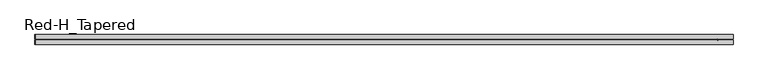
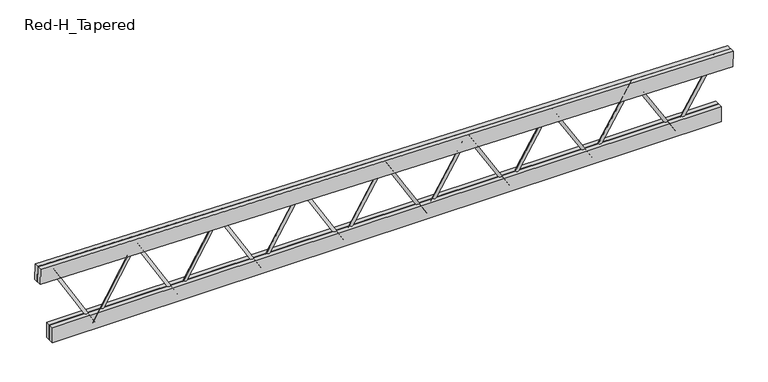
"""IFC4 building model written with IfcOpenShell, lengths in millimetres: beam geometry, Construction_Frames_RedBuilt_Openweb_Red-H_Tapered : Red-H_Tapered."""

from ifc_helpers import new_model, si_unit, point, frame, origin, origin_2d, place, context, project, spatial, polyline, circle_curve, trimmed, segment, composite_curve, outline, extrude, source, transform, mapped, element, save


def red_h_tapered_fac266aa(model_context):
    return source(origin(), model_context, "Body", "SweptSolid", [
        extrude(outline(composite_curve([segment(trimmed(circle_curve(origin_2d(), 12.7), [point((0.0, 12.7))], [point((0.0, -12.7))], False, "CARTESIAN"), True, "CONTINUOUS"), segment(trimmed(circle_curve(origin_2d(), 12.7), [point((0.0, -12.7))], [point((0.0, 12.7))], False, "CARTESIAN"), True, "CONTINUOUS")], self_intersect=False)), frame((2515.0014939, 0.0, -367.0101562), z_axis=(0.5238628746877177, 0.0, 0.8518026112450705), x_axis=(0.0, -1.0, 0.0)), (0.0, 0.0, 1.0), 685.8396444),
        extrude(outline(composite_curve([segment(trimmed(circle_curve(origin_2d(), 12.7), [point((0.0, -12.7000001))], [point((0.0, 12.7))], False, "CARTESIAN"), True, "CONTINUOUS"), segment(trimmed(circle_curve(origin_2d(), 12.7), [point((0.0, 12.7))], [point((0.0, -12.7000001))], False, "CARTESIAN"), True, "CONTINUOUS")], self_intersect=False)), frame((2515.0014939, 0.0, -367.0101562), z_axis=(-0.521291788288458, 0.0, 0.8533785042189788), x_axis=(0.0, -1.0, 0.0)), (0.0, 0.0, 1.0), 689.2223046),
        extrude(outline(composite_curve([segment(trimmed(circle_curve(origin_2d(), 12.7), [point((0.0, 12.7))], [point((0.0, -12.7))], False, "CARTESIAN"), True, "CONTINUOUS"), segment(trimmed(circle_curve(origin_2d(), 12.7), [point((0.0, -12.7))], [point((0.0, 12.7))], False, "CARTESIAN"), True, "CONTINUOUS")], self_intersect=False)), frame((1796.4296385, 0.0, -367.0101562), z_axis=(0.5212917882884571, 0.0, 0.8533785042189793), x_axis=(0.0, -1.0, 0.0)), (0.0, 0.0, 1.0), 689.2223046),
        extrude(outline(composite_curve([segment(trimmed(circle_curve(origin_2d(), 12.7), [point((0.0, -12.7000001))], [point((0.0, 12.6999999))], False, "CARTESIAN"), True, "CONTINUOUS"), segment(trimmed(circle_curve(origin_2d(), 12.7), [point((0.0, 12.6999999))], [point((0.0, -12.7000001))], False, "CARTESIAN"), True, "CONTINUOUS")], self_intersect=False)), frame((1796.4296385, 0.0, -367.0101562), z_axis=(-0.5187411676162772, 0.0, 0.8549313428691812), x_axis=(0.0, -1.0, 0.0)), (0.0, 0.0, 1.0), 692.6111713),
        extrude(outline(composite_curve([segment(trimmed(circle_curve(origin_2d(), 12.7), [point((0.0, 12.7))], [point((0.0, -12.7))], False, "CARTESIAN"), True, "CONTINUOUS"), segment(trimmed(circle_curve(origin_2d(), 12.7), [point((0.0, -12.7))], [point((0.0, 12.7))], False, "CARTESIAN"), True, "CONTINUOUS")], self_intersect=False)), frame((1077.8577831, 0.0, -367.0101562), z_axis=(0.5187411676162762, 0.0, 0.8549313428691818), x_axis=(0.0, -1.0, 0.0)), (0.0, 0.0, 1.0), 692.6111713),
        extrude(outline(composite_curve([segment(trimmed(circle_curve(origin_2d(), 12.7), [point((0.0, -12.7))], [point((0.0, 12.7))], False, "CARTESIAN"), True, "CONTINUOUS"), segment(trimmed(circle_curve(origin_2d(), 12.7), [point((0.0, 12.7))], [point((0.0, -12.7))], False, "CARTESIAN"), True, "CONTINUOUS")], self_intersect=False)), frame((1077.8577831, 0.0, -367.0101562), z_axis=(-0.516210849200197, 0.0, 0.8564615339686958), x_axis=(0.0, -1.0, 0.0)), (0.0, 0.0, 1.0), 696.0061538),
        extrude(outline(composite_curve([segment(trimmed(circle_curve(origin_2d(), 12.7), [point((0.0, 12.7))], [point((0.0, -12.7))], False, "CARTESIAN"), True, "CONTINUOUS"), segment(trimmed(circle_curve(origin_2d(), 12.7), [point((0.0, -12.7))], [point((0.0, 12.7))], False, "CARTESIAN"), True, "CONTINUOUS")], self_intersect=False)), frame((359.2859277, 0.0, -367.0101562), z_axis=(0.5162108492001977, 0.0, 0.8564615339686954), x_axis=(0.0, -1.0, 0.0)), (0.0, 0.0, 1.0), 696.0061538),
        extrude(outline(composite_curve([segment(trimmed(circle_curve(origin_2d(), 12.7), [point((0.0, -12.7))], [point((0.0, 12.6999999))], False, "CARTESIAN"), True, "CONTINUOUS"), segment(trimmed(circle_curve(origin_2d(), 12.7), [point((0.0, 12.6999999))], [point((0.0, -12.7))], False, "CARTESIAN"), True, "CONTINUOUS")], self_intersect=False)), frame((359.2859277, 0.0, -367.0101562), z_axis=(-0.5137006691841284, 0.0, 0.857969476426626), x_axis=(0.0, -1.0, 0.0)), (0.0, 0.0, 1.0), 699.4071631),
        extrude(outline(composite_curve([segment(trimmed(circle_curve(origin_2d(), 12.7), [point((0.0, -12.6999999))], [point((0.0, 12.7))], False, "CARTESIAN"), True, "CONTINUOUS"), segment(trimmed(circle_curve(origin_2d(), 12.7), [point((0.0, 12.7))], [point((0.0, -12.6999999))], False, "CARTESIAN"), True, "CONTINUOUS")], self_intersect=False)), frame((-359.2859277, 0.0, -367.0101562), z_axis=(0.5137006691840971, 0.0, 0.8579694764266448), x_axis=(0.0, -1.0, 0.0)), (0.0, 0.0, 1.0), 699.4071631),
        extrude(outline(composite_curve([segment(trimmed(circle_curve(origin_2d(), 12.7), [point((0.0, 12.6999999))], [point((0.0, -12.7))], False, "CARTESIAN"), True, "CONTINUOUS"), segment(trimmed(circle_curve(origin_2d(), 12.7), [point((0.0, -12.7))], [point((0.0, 12.6999999))], False, "CARTESIAN"), True, "CONTINUOUS")], self_intersect=False)), frame((-359.2859277, 0.0, -367.0101562), z_axis=(-0.5112104634271143, 0.0, 0.8594555614356307), x_axis=(0.0, -1.0, 0.0)), (0.0, 0.0, 1.0), 702.8141116),
        extrude(outline(composite_curve([segment(trimmed(circle_curve(origin_2d(), 12.7), [point((0.0, -12.6999999))], [point((0.0, 12.7000001))], False, "CARTESIAN"), True, "CONTINUOUS"), segment(trimmed(circle_curve(origin_2d(), 12.7), [point((0.0, 12.7000001))], [point((0.0, -12.6999999))], False, "CARTESIAN"), True, "CONTINUOUS")], self_intersect=False)), frame((-1077.8577831, 0.0, -367.0101562), z_axis=(0.5112104634271127, 0.0, 0.8594555614356316), x_axis=(0.0, -1.0, 0.0)), (0.0, 0.0, 1.0), 702.8141116),
        extrude(outline(composite_curve([segment(trimmed(circle_curve(origin_2d(), 12.7), [point((0.0, 12.7))], [point((0.0, -12.7))], False, "CARTESIAN"), True, "CONTINUOUS"), segment(trimmed(circle_curve(origin_2d(), 12.7), [point((0.0, -12.7))], [point((0.0, 12.7))], False, "CARTESIAN"), True, "CONTINUOUS")], self_intersect=False)), frame((-1077.8577831, 0.0, -367.0101562), z_axis=(-0.5087400675988082, 0.0, 0.8609201726173921), x_axis=(0.0, -1.0, 0.0)), (0.0, 0.0, 1.0), 706.2269135),
        extrude(outline(composite_curve([segment(trimmed(circle_curve(origin_2d(), 12.7), [point((0.0, -12.7))], [point((0.0, 12.7))], False, "CARTESIAN"), True, "CONTINUOUS"), segment(trimmed(circle_curve(origin_2d(), 12.7), [point((0.0, 12.7))], [point((0.0, -12.7))], False, "CARTESIAN"), True, "CONTINUOUS")], self_intersect=False)), frame((-1796.4296385, 0.0, -367.0101562), z_axis=(0.5087400675988213, 0.0, 0.8609201726173843), x_axis=(0.0, -1.0, 0.0)), (0.0, 0.0, 1.0), 706.2269135),
        extrude(outline(composite_curve([segment(trimmed(circle_curve(origin_2d(), 12.7), [point((0.0, 12.7))], [point((0.0, -12.7))], False, "CARTESIAN"), True, "CONTINUOUS"), segment(trimmed(circle_curve(origin_2d(), 12.7), [point((0.0, -12.7))], [point((0.0, 12.7))], False, "CARTESIAN"), True, "CONTINUOUS")], self_intersect=False)), frame((-1796.4296385, 0.0, -367.0101562), z_axis=(-0.5062893172698196, 0.0, 0.8623636861663762), x_axis=(0.0, -1.0, 0.0)), (0.0, 0.0, 1.0), 709.6454842),
        extrude(outline(composite_curve([segment(trimmed(circle_curve(origin_2d(), 12.7), [point((0.0, -12.7))], [point((0.0, 12.7000001))], False, "CARTESIAN"), True, "CONTINUOUS"), segment(trimmed(circle_curve(origin_2d(), 12.7), [point((0.0, 12.7000001))], [point((0.0, -12.7))], False, "CARTESIAN"), True, "CONTINUOUS")], self_intersect=False)), frame((-2515.0014939, 0.0, -367.0101562), z_axis=(0.506289317269808, 0.0, 0.862363686166383), x_axis=(0.0, -1.0, 0.0)), (0.0, 0.0, 1.0), 709.6454842),
        extrude(outline(composite_curve([segment(trimmed(circle_curve(origin_2d(), 12.7), [point((0.0, 12.7))], [point((0.0, -12.7))], False, "CARTESIAN"), True, "CONTINUOUS"), segment(trimmed(circle_curve(origin_2d(), 12.7), [point((0.0, -12.7))], [point((0.0, 12.7))], False, "CARTESIAN"), True, "CONTINUOUS")], self_intersect=False)), frame((-2515.0014939, 0.0, -367.0101562), z_axis=(-0.5038580479976326, 0.0, 0.8637864709915382), x_axis=(0.0, -1.0, 0.0)), (0.0, 0.0, 1.0), 713.0697408),
        extrude(outline(polyline([(-2899.6874215, -41.275), (-2899.6874215, -3.175), (2899.6874215, -3.175), (2899.6874215, -41.275), (-2899.6874215, -41.275)])), frame((0.0, 0.0, -386.0601562), z_axis=(0.0, 0.0, 1.0), x_axis=(1.0, 0.0, 0.0)), (0.0, 0.0, 1.0), 139.7),
        extrude(outline(polyline([(-2899.6874215, 3.175), (-2899.6874215, 41.275), (2899.6874215, 41.275), (2899.6874215, 3.175), (-2899.6874215, 3.175)])), frame((0.0, 0.0, -386.0601562), z_axis=(0.0, 0.0, 1.0), x_axis=(1.0, 0.0, 0.0)), (0.0, 0.0, 1.0), 139.7),
        extrude(outline(polyline([(0.0, -38.1), (0.0, 0.0), (6003.4346259, 0.0), (6003.4346259, -38.1), (0.0, -38.1)])), frame((-3003.6516548, -3.175, 185.4598509), z_axis=(0.01692364560154581, 0.0, 0.9998567848544877), x_axis=(0.9998567848544877, 0.0, -0.01692364560154581)), (0.0, 0.0, 1.0), 139.7),
        extrude(outline(polyline([(0.0, -38.1), (0.0, 0.0), (6003.4346259, 0.0), (6003.4346259, -38.1), (0.0, -38.1)])), frame((-3003.6516548, 41.275, 185.4598509), z_axis=(0.01692364560154581, 0.0, 0.9998567848544877), x_axis=(0.9998567848544877, 0.0, -0.01692364560154581)), (0.0, 0.0, 1.0), 139.7),
    ])


if __name__ == "__main__":
    model = new_model("IFC4")
    model_context = context("Model", 3, world=origin())
    ifc_project = project(units=[si_unit("LENGTHUNIT", "METRE", prefix="MILLI")], contexts=[model_context])
    site = spatial("IfcSite", under=ifc_project)
    building = spatial("IfcBuilding", under=site)
    placement = place(None, origin())
    red_h_tapered_shape = red_h_tapered_fac266aa(model_context)
    element("IfcBeam", 1, ObjectType="Construction_Frames_RedBuilt_Openweb_Red-H_Tapered : Red-H_Tapered", at=placement, inside=building, context=model_context, shape_type="MappedRepresentation", body=[
        mapped(red_h_tapered_shape, transform((0.0, 0.0, 0.0), x_axis=(1.0, 0.0, 0.0), y_axis=(0.0, 1.0, 0.0), z_axis=(0.0, 0.0, 1.0))),
    ])
    save(model, "model.ifc")

# Revit data of these elements
# Type "Construction_Frames_RedBuilt_Openweb_Red-H_Tapered : Red-H_Tapered"
#   Youtube clip = ""
#   Weight Net (Kg) = "0"
#   Webs = "Up to 2\" diameter tubular steel"
#   Uniformat II Description = ""
#   Uniformat II Code = ""
#   Uniclass 2015 Name = "Softwood trusses"
#   Uniclass 2015 Code = "Pr_20_85_90_81"
#   Uniclass 2.0 Description = "Structural Framing Systems"
#   Uniclass 2.0 Code = "SS-15-10-75"
#   Uniclass 1.4 Description = "Trusses"
#   Uniclass 1.4 Code = "L3523"
#   UNSPSC Code = "30103606"
#   Technical description = "http://www.redbuilt.com/reference/literature-and-other-resources"
#   Region South America = "None"
#   Region Oceania = "None"
#   Region North America = "US"
#   Region Middle East = "None"
#   Region Europe = "None"
#   Region Asia = "None"
#   Region Antarctica = "None"
#   Region Africa = "None"
#   QR code = "http://bimobject.com/redbuilt/product/redbuilt-0003"
#   Product url = "http://www.redbuilt.com/products/default.aspx?id=2"
#   Product group = "Wood Trusses"
#   Product family = "Construction"
#   Product data url = "https://bimobject.com/redbuilt/product/redbuilt-0003"
#   Product certification = ""
#   Product SKU = "redbuilt-0003"
#   Product Page URL = "http://www.redbuilt.com/commercial-systems/red-m-red-h-open-web-trusses"
#   Product Guid = "2c5793f2-6ffb-4665-b825-cf90c048e711"
#   Product Documentation Link = "http://www.redbuilt.com/documents/OW_Guide_2017_07_LowRes_wLinks.pdf"
#   OmniClass Description = "Wood Trusses"
#   OmniClass Code = "23-13 35 19 13 17"
#   NBS Reference Description = ""
#   NBS Reference Code = ""
#   Material secondary = "Steel"
#   Material main = "CHARRED WOOD"
#   Masterformat 2014 Description = "Metal-Web Wood Joists"
#   Masterformat 2014 Code = "06 17 36"
#   Manufacturer name = "RedBuilt"
#   Manufacturer country = "United States"
#   Installation instructions = "http://www.redbuilt.com/documents/Installation_Sheets_Open-Web.pdf"
#   IFC Classification = ""
#   EAN code = ""
#   Design country = "United States"
#   Product Information = "http://redbuilt.com/products/default.aspx?id=2"
#   Model = "Red-H-Tapered"
#   Manufacturer URL = "http://redbuilt.com/"
#   Manufacturer = "RedBuilt™"
#   Description = "Open Web Truss"
#   Date of publishing = "8/17/2010"
#   Contact us = "http://redbuilt.com/contact/"
#   Chords = "Double 1½\" x 5½\" MSR lumber"
#   COBIe Type Category = ""
#   Brand url = "http://www.redbuilt.com"
#   BIMobject main category code = "construction"
#   BIMobject main category = "Construction"
#   BIMobject category code = "construction-frames-trusses"
#   BIMobject category = "Frames & Trusses"
#   Web Radius = 0' - 0 1/2"
#   Web Layout Offset Start [instance default] = 0' - 5"
#   Web Layout Offset End [instance default] = 0' - 5"
#   Web Diameter = 0' - 1"
#   TotalLength [instance default] = 20' - 0"
#   Span Minimum = 4' - 0"
#   Span Maximum = 70' - 0"
#   Span Limit [instance default] = 20' - 0"
#   Nominal width = 0' - 0"
#   Nominal height = 0' - 0"
#   Inner Depth Top [instance default] = 0' - 2.76372"
#   Depth Start [instance default] = 6' - 0"
#   Top Chord Length [instance default] = 20' - 1.19701"
#   TC Extension Start Aux [instance default] = 0' - 0"
#   TC Extension End Aux [instance default] = 0' - 0"
#   T-B Chord Length Difference L [instance default] = 0' - 4"
#   T-B Chord Length Difference [instance default] = 0' - 4"
#   Height 2 [instance default] = 6' - 0"
#   Depth Minimum at Wall = 2' - 0"
#   Depth Maximum at Wall = 6' - 0"
#   Depth Lower End [instance default] = 2' - 0"
#   Depth Higher End [instance default] = 6' - 0"
#   Depth End [instance default] = 2' - 0"
#   Depth 2 [instance default] = 2' - 0"
#   Chord Width = 0' - 3 1/4"
#   Chord Thickness = 0' - 1 1/2"
#   Chord Depth = 0' - 5 1/2"
#   Offset Start [instance default] = 0' - 0"
#   TC Extension Start [instance default] = 0' - 0"
#   End Panel = 0' - 5"
#   Offset End [instance default] = 0' - 0"
#   TC Extension End [instance default] = 0' - 0"
#   Length [instance default] = 20' - 0"
#   Angle [instance default] = 5.71059°
#   Span Limit Warning [instance default] = no
#   Edition number = 1
#   Top Bearing Start [instance default] = yes
#   Top Bearing End [instance default] = yes
#   Bottom Bearing Start [instance default] = no
#   Bottom Bearing End [instance default] = no
#   8 Panels [instance default] = yes
#   16 Panels [instance default] = no
#   12 Panels [instance default] = no
#   Web Material = RedBuilt-Steel, Galvanized
#   Clip Material = RedBuilt-Steel, Galvanized
#   Chords Material = WOOD-OAKFIRE
#   URL = ""
#   Assembly Code = ""
# Element 1 (IfcBeam, "Construction_Frames_RedBuilt_Openweb_Red-H_Tapered : Red-H_Tapered")
#   TotalLength = 19' - 8.32184"
#   Span Limit = 19' - 8.32184"
#   Inner Depth Top = 0' - 2.75039"
#   Depth Start = 5' - 0"
#   Top Chord Length = 19' - 8.35569"
#   Height 2 = 5' - 0"
#   Depth Higher End = 5' - 0"
#   Depth 2 = 0' - 4"
#   Angle = 0.9697°
#   Materials on its faces: "RedBuilt-Steel, Galvanized", "WOOD-OAKFIRE"
# Materials
#   "RedBuilt-Steel, Galvanized": class "Metal", colour RGB 164 172 176, transparency 0, Manufacturer = "RedBuilt. LLC", Comments = "Openweb Metal Web", URL = "http://www.redbuilt.com/", Description = "Galvanized steel", Cost = 0
#   "WOOD-OAKFIRE": class "Wood", colour RGB 198 202 183, transparency 0, Description = "Generic wood", Cost = 0
